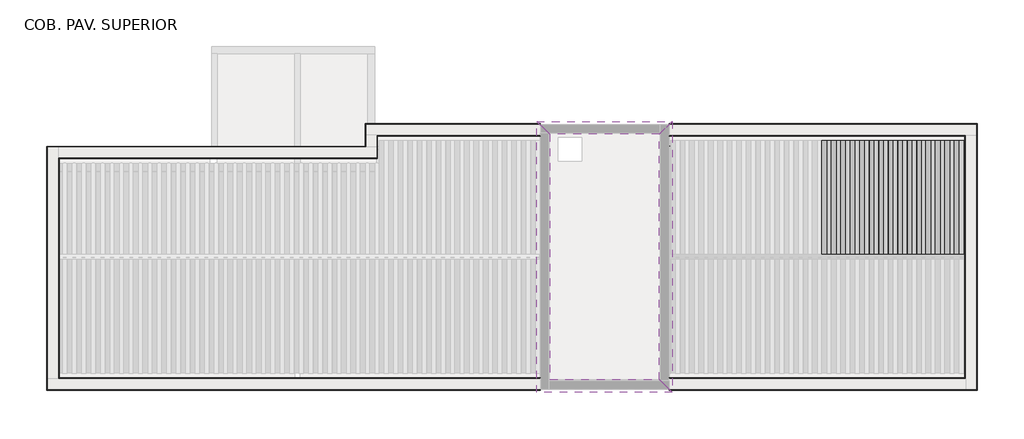
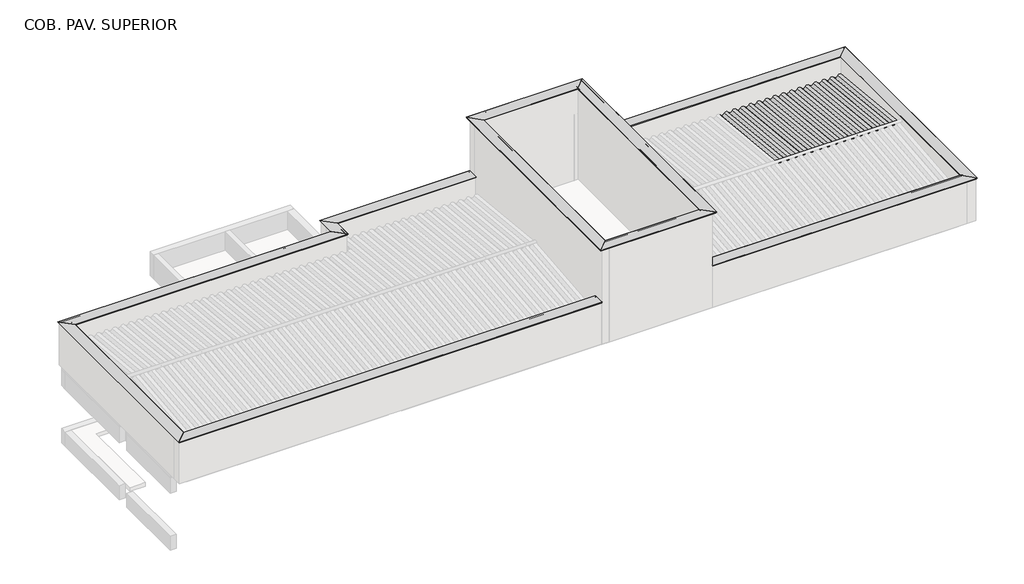
# One storey, part 7 of 7: 25 beams, 9 columns, 4 proxies.
# Revit data of these elements (continued)
# Type "Madeira de lei : Berço 6x12cm"
#   A = 0.02 m²
#   Length [instance default] = 1.524 m
#   b = 0.06 m
#   d = 0.12 m
#   Structural Material [instance default] = none
#   Assembly Code = ""
# Type "TQS - Viga retangular : 19.0 x 80.0"
#   Length [instance default] = 1.524 m
#   b = 0.19 m
#   h = 0.80 m
#   Structural Material [instance default] = none
#   Assembly Code = ""
# Type "Telha Ondulada : Fibrocimento"
#   Description = "TELHA ONDULADA FIBROCIMENTO"
#   Cost = 5
#   Length [instance default] = 1.524 m
#   b = 0.07 m
#   h = 0.16 m
#   Structural Material = .TELHA DE FIBROCIMENTO
#   Assembly Code = ""
# Type ".CC_RUFO_PINGADEIRA_27 cm"
#   Description = "RUFO METÁLICO"
# Type "Madeira de lei-Coluna : Pontalete 6X16cm"
#   A = 0.01952 m²
#   b = 0.06 m
#   d = 0.16 m
#   Structural Material [instance default] = none
#   Assembly Code = ""
# Elements 1, 2, 3, 4, 5, 6, 7, 8 (IfcBeam, "Madeira de lei : Berço 6x12cm")
#   Comments = ""
#   Structural Material = .MADEIRAMENTO
#   Phase Created = CC_PE
#   Materials on its faces: ".MADEIRAMENTO"
# Element 9 (IfcBeam, "TQS - Viga retangular : 19.0 x 80.0")
#   Uso = "ESTRUTURA"
#   Titulo = "V420"
#   Chave = "-396"
#   Tipo Elemento = "Viga"
#   SHA1 = "BF00FA4722BD5D14A0B3A55AFD137769A58BF563"
#   Revisão = ""
#   Tipo de carga = ""
#   Divisor de flexao = ""
#   Secao = ""
#   Configuracao = ""
#   Angulo (graus) = ""
#   Detalhamento = ""
#   Casos de vento manual = ""
#   Tipo = ""
#   Alcas = ""
#   Furos = ""
#   Pino = ""
#   Distribuicao = ""
#   Solidarizado = ""
#   Solidarizar na montagem = ""
#   Unir com o próximo = ""
#   Grupo pre moldado = ""
#   Verificado = ""
#   Concreto C = ""
#   Taxa de armadura (kgf/m³) = 0
#   Carga (tf/m²) = 0
#   Carga (tf/m) = 0
#   Carga (tf) = 0
#   Altura = 0.80 m
#   Rebaixo = -0.60 m
#   Largura = 0.19 m
#   Distancia a face = 0.00 m
#   Distancia ao eixo = 0.00 m
#   Altura gerber esquerda = 0.00 m
#   Largura gerber esquerda = 0.00 m
#   Altura gerber direita = 0.00 m
#   Largura gerber direita = 0.00 m
#   Resultado de Ensaios fck (MPa) = 0
#   Unique TQS ID = -396
#   Principal = yes
#   Structural Material = none
#   Phase Created = CC_PE
# Element 10 (IfcBeam, "TQS - Viga retangular : 19.0 x 80.0")
#   Uso = "ESTRUTURA"
#   Titulo = "V403"
#   Chave = "-414"
#   Tipo Elemento = "Viga"
#   SHA1 = "CAFE63EDCF06386714B4FC392C56034EE987500E"
#   Revisão = ""
#   Tipo de carga = ""
#   Divisor de flexao = ""
#   Secao = ""
#   Configuracao = ""
#   Angulo (graus) = ""
#   Detalhamento = ""
#   Casos de vento manual = ""
#   Tipo = ""
#   Alcas = ""
#   Furos = ""
#   Pino = ""
#   Distribuicao = ""
#   Solidarizado = ""
#   Solidarizar na montagem = ""
#   Unir com o próximo = ""
#   Grupo pre moldado = ""
#   Verificado = ""
#   Concreto C = ""
#   Taxa de armadura (kgf/m³) = 0
#   Carga (tf/m²) = 0
#   Carga (tf/m) = 0
#   Carga (tf) = 0
#   Altura = 0.80 m
#   Rebaixo = -0.60 m
#   Largura = 0.19 m
#   Distancia a face = 0.00 m
#   Distancia ao eixo = 0.00 m
#   Altura gerber esquerda = 0.00 m
#   Largura gerber esquerda = 0.00 m
#   Altura gerber direita = 0.00 m
#   Largura gerber direita = 0.00 m
#   Resultado de Ensaios fck (MPa) = 0
#   Unique TQS ID = -414
#   Principal = yes
#   Structural Material = none
#   Phase Created = CC_PE
# Elements 11, 12, 13, 14, 15, 16, 17, 18, 19, 20, 21, 22, 23, 24, 25 (IfcBeam, "Telha Ondulada : Fibrocimento")
#   Phase Created = CC_PE
#   Materials on its faces: ".TELHA DE FIBROCIMENTO"
# Element 26 (IfcBuildingElementProxy, ".CC_RUFO_PINGADEIRA_27 cm")
#   Uso = "RUFOS COB. PAV. SUPERIOR"
#   Phase Created = CC_PE
#   Materials on its faces: ".ALUMÍNIO COM PINTURA LÁTEX BRANCA"
# Elements 27, 28, 29 (IfcBuildingElementProxy, ".CC_RUFO_PINGADEIRA_27 cm")
#   Uso = "RUFOS COB. CAIXA D'ÁGUA"
#   Phase Created = CC_PE
#   Materials on its faces: ".ALUMÍNIO COM PINTURA LÁTEX BRANCA"
# Elements 30, 31, 32, 33, 34, 35, 36, 37, 38 (IfcColumn, "Madeira de lei-Coluna : Pontalete 6X16cm")
#   Comments = ""
#   Structural Material = .MADEIRAMENTO
#   Phase Created = CC_PE
#   Materials on its faces: ".MADEIRAMENTO"
# Materials
#   ".TELHA DE FIBROCIMENTO": class "CC_TELHADO", colour RGB 77 77 76, transparency 0, Description = "TELHA ONDULADA FIBROCIMENTO", Cost = 0
#   ".MADEIRAMENTO": class ".CC_MADEIRAS", colour RGB 212 179 113, transparency 0, Cost = 0
#   ".ALUMÍNIO COM PINTURA LÁTEX BRANCA": class "Generic", colour RGB 250 250 250, transparency 0, Cost = 0
